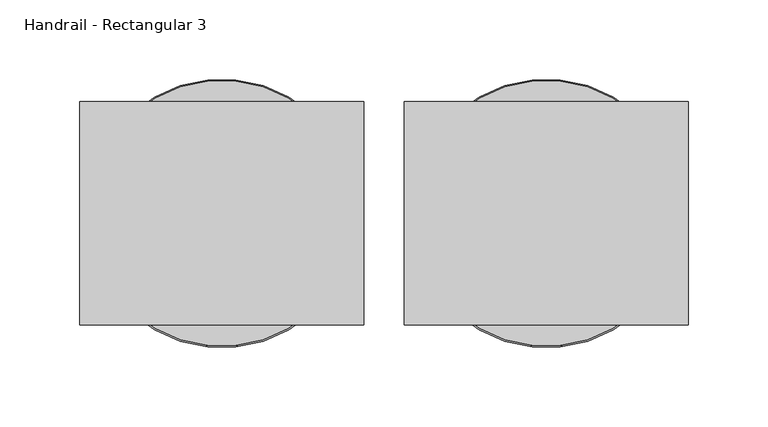
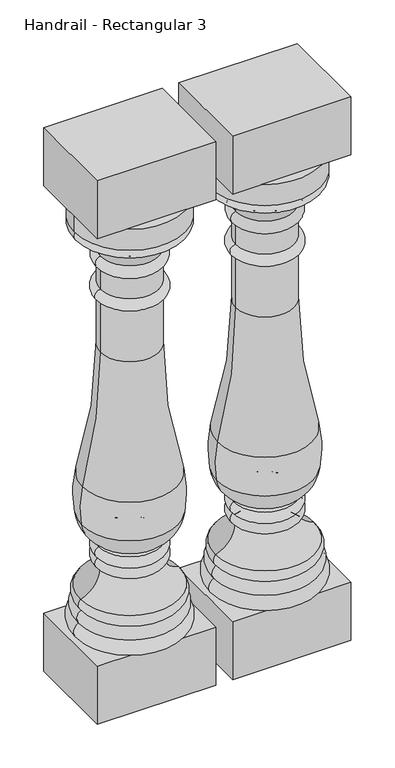
"""IFC4 building model written with IfcOpenShell, lengths in millimetres: railing geometry, Handrail - Rectangular 3."""

from ifc_helpers import new_model, si_unit, point, frame, origin, place, context, project, spatial, polyline, circle_curve, ellipse_curve, trimmed, outline, extrude, source, transform, mapped, element, save
from ifc_brep_helpers import plane_surface, cylinder_surface, revolved_surface, advanced_brep


def handrail_rectangular_3_6060ea51(model_context):
    return source(origin(), model_context, "Body", "SolidModel", [
        advanced_brep(
        [(11610.7084395, -1665.6164768, 849.3125), (11777.3959395, -1665.6164768, 849.3125), (11777.3959395, -1665.6164768, 882.65), (11610.7084395, -1665.6164768, 882.65), (11613.8834395, -1665.6164768, 849.3125), (11774.2209395, -1665.6164768, 849.3125), (11613.8834395, -1665.6164768, 835.025), (11774.2209395, -1665.6164768, 835.025), (11650.3959395, -1665.6164768, 796.925), (11737.7084395, -1665.6164768, 796.925), (11650.3959395, -1665.6164768, 777.875), (11737.7084395, -1665.6164768, 777.875), (11650.3959395, -1665.6164768, 744.5375), (11737.7084395, -1665.6164768, 744.5375), (11650.3959395, -1665.6164768, 727.075), (11737.7084395, -1665.6164768, 727.075), (11650.3959395, -1665.6164768, 644.525), (11737.7084395, -1665.6164768, 644.525), (11623.2074221, -1665.6164768, 440.2065586), (11764.896957, -1665.6164768, 440.2065586), (11622.0170661, -1665.6164768, 379.6643134), (11766.087313, -1665.6164768, 379.6643134), (11649.2281246, -1665.6164768, 340.8286685), (11738.8762545, -1665.6164768, 340.8286685), (11647.5028429, -1665.6164768, 336.3463085), (11740.6015362, -1665.6164768, 336.3463085), (11646.4271895, -1665.6164768, 319.0875), (11741.6771895, -1665.6164768, 319.0875), (11649.6021895, -1665.6164768, 301.625), (11738.5021895, -1665.6164768, 301.625), (11620.2334395, -1665.6164768, 261.9375), (11767.8709395, -1665.6164768, 261.9375), (11621.0271895, -1665.6164768, 244.475), (11767.0771895, -1665.6164768, 244.475), (11617.0584395, -1665.6164768, 225.425), (11771.0459395, -1665.6164768, 225.425), (11613.8834395, -1665.6164768, 203.2), (11774.2209395, -1665.6164768, 203.2), (11694.0521895, -1665.6164768, 203.2), (11694.0521895, -1665.6164768, 882.65)],
        [
            (0, 1, circle_curve(frame((11694.0521895, -1665.6164768, 849.3125), z_axis=(0.0, 0.0, 1.0), x_axis=(1.0, 0.0, 0.0)), 83.34375)),
            (1, 2),
            (2, 3, circle_curve(frame((11694.0521895, -1665.6164768, 882.65), z_axis=(0.0, 0.0, -1.0), x_axis=(1.0, 0.0, 0.0)), 83.34375)),
            (3, 0),
            (1, 0, circle_curve(frame((11694.0521895, -1665.6164768, 849.3125), z_axis=(0.0, 0.0, 1.0), x_axis=(1.0, 0.0, 0.0)), 83.34375)),
            (3, 2, circle_curve(frame((11694.0521895, -1665.6164768, 882.65), z_axis=(0.0, 0.0, -1.0), x_axis=(1.0, 0.0, 0.0)), 83.34375)),
            (4, 5, circle_curve(frame((11694.0521895, -1665.6164768, 849.3125), z_axis=(0.0, 0.0, 1.0), x_axis=(1.0, 0.0, 0.0)), 80.16875)),
            (5, 1),
            (0, 4),
            (5, 4, circle_curve(frame((11694.0521895, -1665.6164768, 849.3125), z_axis=(0.0, 0.0, 1.0), x_axis=(1.0, 0.0, 0.0)), 80.16875)),
            (6, 7, circle_curve(frame((11694.0521895, -1665.6164768, 835.025), z_axis=(0.0, 0.0, 1.0), x_axis=(1.0, 0.0, 0.0)), 80.16875)),
            (7, 5, circle_curve(frame((11767.7717208, -1665.6164768, 842.16875), z_axis=(0.0, -1.0, 0.0), x_axis=(1.0, 0.0, 0.0)), 9.6242187)),
            (4, 6, circle_curve(frame((11620.3326583, -1665.6164768, 842.16875), z_axis=(0.0, -1.0, 0.0), x_axis=(-1.0, 0.0, 0.0)), 9.6242187)),
            (7, 6, circle_curve(frame((11694.0521895, -1665.6164768, 835.025), z_axis=(0.0, 0.0, 1.0), x_axis=(1.0, 0.0, 0.0)), 80.16875)),
            (8, 9, circle_curve(frame((11694.0521895, -1665.6164768, 796.925), z_axis=(0.0, 0.0, 1.0), x_axis=(1.0, 0.0, 0.0)), 43.65625)),
            (9, 7, circle_curve(frame((11793.125244, -1665.6164768, 780.362802), z_axis=(0.0, 1.0, 0.0), x_axis=(1.0, 0.0, 0.0)), 57.8388159)),
            (6, 8, circle_curve(frame((11594.9791351, -1665.6164768, 780.362802), z_axis=(0.0, 1.0, 0.0), x_axis=(-1.0, 0.0, 0.0)), 57.8388159)),
            (9, 8, circle_curve(frame((11694.0521895, -1665.6164768, 796.925), z_axis=(0.0, 0.0, 1.0), x_axis=(1.0, 0.0, 0.0)), 43.65625)),
            (10, 11, circle_curve(frame((11694.0521895, -1665.6164768, 777.875), z_axis=(0.0, 0.0, 1.0), x_axis=(1.0, 0.0, 0.0)), 43.65625)),
            (11, 9, circle_curve(frame((11735.9621895, -1665.6164768, 787.4), z_axis=(0.0, -1.0, 0.0), x_axis=(1.0, 0.0, 0.0)), 9.68375)),
            (8, 10, circle_curve(frame((11652.1421895, -1665.6164768, 787.4), z_axis=(0.0, -1.0, 0.0), x_axis=(-1.0, 0.0, 0.0)), 9.68375)),
            (11, 10, circle_curve(frame((11694.0521895, -1665.6164768, 777.875), z_axis=(0.0, 0.0, 1.0), x_axis=(1.0, 0.0, 0.0)), 43.65625)),
            (12, 13, circle_curve(frame((11694.0521895, -1665.6164768, 744.5375), z_axis=(0.0, 0.0, 1.0), x_axis=(1.0, 0.0, 0.0)), 43.65625)),
            (13, 11),
            (10, 12),
            (13, 12, circle_curve(frame((11694.0521895, -1665.6164768, 744.5375), z_axis=(0.0, 0.0, 1.0), x_axis=(1.0, 0.0, 0.0)), 43.65625)),
            (14, 15, circle_curve(frame((11694.0521895, -1665.6164768, 727.075), z_axis=(0.0, 0.0, 1.0), x_axis=(1.0, 0.0, 0.0)), 43.65625)),
            (15, 13, circle_curve(frame((11737.7084395, -1665.6164768, 735.80625), z_axis=(0.0, -1.0, 0.0), x_axis=(1.0, 0.0, 0.0)), 8.73125)),
            (12, 14, circle_curve(frame((11650.3959395, -1665.6164768, 735.80625), z_axis=(0.0, -1.0, 0.0), x_axis=(-1.0, 0.0, 0.0)), 8.73125)),
            (15, 14, circle_curve(frame((11694.0521895, -1665.6164768, 727.075), z_axis=(0.0, 0.0, 1.0), x_axis=(1.0, 0.0, 0.0)), 43.65625)),
            (16, 17, circle_curve(frame((11694.0521895, -1665.6164768, 644.525), z_axis=(0.0, 0.0, 1.0), x_axis=(1.0, 0.0, 0.0)), 43.65625)),
            (17, 15),
            (14, 16),
            (17, 16, circle_curve(frame((11694.0521895, -1665.6164768, 644.525), z_axis=(0.0, 0.0, 1.0), x_axis=(1.0, 0.0, 0.0)), 43.65625)),
            (18, 19, circle_curve(frame((11694.0521895, -1665.6164768, 440.2065586), z_axis=(0.0, 0.0, 1.0), x_axis=(1.0, 0.0, 0.0)), 70.8447675)),
            (19, 17, circle_curve(frame((12472.4851891, -1665.6164768, 638.333048), z_axis=(0.0, 1.0, 0.0), x_axis=(1.0, 0.0, 0.0)), 734.8028389)),
            (16, 18, circle_curve(frame((10915.61919, -1665.6164768, 638.333048), z_axis=(0.0, 1.0, 0.0), x_axis=(-1.0, 0.0, 0.0)), 734.8028389)),
            (19, 18, circle_curve(frame((11694.0521895, -1665.6164768, 440.2065586), z_axis=(0.0, 0.0, 1.0), x_axis=(1.0, 0.0, 0.0)), 70.8447675)),
            (20, 21, circle_curve(frame((11694.0521895, -1665.6164768, 379.6643134), z_axis=(0.0, 0.0, 1.0), x_axis=(1.0, 0.0, 0.0)), 72.0351235)),
            (21, 19, circle_curve(frame((11606.9983349, -1665.6164768, 406.819198), z_axis=(0.0, -1.0, 0.0), x_axis=(1.0, 0.0, 0.0)), 161.3898718)),
            (18, 20, circle_curve(frame((11781.1060442, -1665.6164768, 406.819198), z_axis=(0.0, -1.0, 0.0), x_axis=(-1.0, 0.0, 0.0)), 161.3898718)),
            (21, 20, circle_curve(frame((11694.0521895, -1665.6164768, 379.6643134), z_axis=(0.0, 0.0, 1.0), x_axis=(1.0, 0.0, 0.0)), 72.0351235)),
            (22, 23, circle_curve(frame((11694.0521895, -1665.6164768, 340.8286685), z_axis=(0.0, 0.0, 1.0), x_axis=(1.0, 0.0, 0.0)), 44.8240649)),
            (23, 21, circle_curve(frame((11716.3572912, -1665.6164768, 385.5579203), z_axis=(0.0, -1.0, 0.0), x_axis=(1.0, 0.0, 0.0)), 50.0780358)),
            (20, 22, circle_curve(frame((11671.7470879, -1665.6164768, 385.5579203), z_axis=(0.0, -1.0, 0.0), x_axis=(-1.0, 0.0, 0.0)), 50.0780358)),
            (23, 22, circle_curve(frame((11694.0521895, -1665.6164768, 340.8286685), z_axis=(0.0, 0.0, 1.0), x_axis=(1.0, 0.0, 0.0)), 44.8240649)),
            (24, 25, circle_curve(frame((11694.0521895, -1665.6164768, 336.3463085), z_axis=(0.0, 0.0, 1.0), x_axis=(1.0, 0.0, 0.0)), 46.5493467)),
            (25, 23, circle_curve(frame((11741.6771895, -1665.6164768, 339.3335472), z_axis=(0.0, 1.0, 0.0), x_axis=(1.0, 0.0, 0.0)), 3.175)),
            (22, 24, circle_curve(frame((11646.4271895, -1665.6164768, 339.3335472), z_axis=(0.0, 1.0, 0.0), x_axis=(-1.0, 0.0, 0.0)), 3.175)),
            (25, 24, circle_curve(frame((11694.0521895, -1665.6164768, 336.3463085), z_axis=(0.0, 0.0, 1.0), x_axis=(1.0, 0.0, 0.0)), 46.5493467)),
            (26, 27, circle_curve(frame((11694.0521895, -1665.6164768, 319.0875), z_axis=(0.0, 0.0, 1.0), x_axis=(1.0, 0.0, 0.0)), 47.625)),
            (27, 25, circle_curve(frame((11736.6008248, -1665.6164768, 327.4340404), z_axis=(0.0, -1.0, 0.0), x_axis=(1.0, 0.0, 0.0)), 9.7690437)),
            (24, 26, circle_curve(frame((11651.5035543, -1665.6164768, 327.4340404), z_axis=(0.0, -1.0, 0.0), x_axis=(-1.0, 0.0, 0.0)), 9.7690437)),
            (27, 26, circle_curve(frame((11694.0521895, -1665.6164768, 319.0875), z_axis=(0.0, 0.0, 1.0), x_axis=(1.0, 0.0, 0.0)), 47.625)),
            (28, 29, circle_curve(frame((11694.0521895, -1665.6164768, 301.625), z_axis=(0.0, 0.0, 1.0), x_axis=(1.0, 0.0, 0.0)), 44.45)),
            (29, 27, circle_curve(frame((11737.0635177, -1665.6164768, 310.9064631), z_axis=(0.0, -1.0, 0.0), x_axis=(1.0, 0.0, 0.0)), 9.3923018)),
            (26, 28, circle_curve(frame((11651.0408614, -1665.6164768, 310.9064631), z_axis=(0.0, -1.0, 0.0), x_axis=(-1.0, 0.0, 0.0)), 9.3923018)),
            (29, 28, circle_curve(frame((11694.0521895, -1665.6164768, 301.625), z_axis=(0.0, 0.0, 1.0), x_axis=(1.0, 0.0, 0.0)), 44.45)),
            (30, 31, circle_curve(frame((11694.0521895, -1665.6164768, 261.9375), z_axis=(0.0, 0.0, 1.0), x_axis=(1.0, 0.0, 0.0)), 73.81875)),
            (31, 29, circle_curve(frame((11780.0024429, -1665.6164768, 301.625), z_axis=(0.0, 1.0, 0.0), x_axis=(1.0, 0.0, 0.0)), 41.5002534)),
            (28, 30, circle_curve(frame((11608.1019362, -1665.6164768, 301.625), z_axis=(0.0, 1.0, 0.0), x_axis=(-1.0, 0.0, 0.0)), 41.5002534)),
            (31, 30, circle_curve(frame((11694.0521895, -1665.6164768, 261.9375), z_axis=(0.0, 0.0, 1.0), x_axis=(1.0, 0.0, 0.0)), 73.81875)),
            (32, 33, circle_curve(frame((11694.0521895, -1665.6164768, 244.475), z_axis=(0.0, 0.0, 1.0), x_axis=(1.0, 0.0, 0.0)), 73.025)),
            (33, 31, circle_curve(frame((11758.5664257, -1665.6164768, 253.6111427), z_axis=(0.0, -1.0, 0.0), x_axis=(1.0, 0.0, 0.0)), 12.4860804)),
            (30, 32, circle_curve(frame((11629.5379534, -1665.6164768, 253.6111427), z_axis=(0.0, -1.0, 0.0), x_axis=(-1.0, 0.0, 0.0)), 12.4860804)),
            (33, 32, circle_curve(frame((11694.0521895, -1665.6164768, 244.475), z_axis=(0.0, 0.0, 1.0), x_axis=(1.0, 0.0, 0.0)), 73.025)),
            (34, 35, circle_curve(frame((11694.0521895, -1665.6164768, 225.425), z_axis=(0.0, 0.0, 1.0), x_axis=(1.0, 0.0, 0.0)), 76.99375)),
            (35, 33, circle_curve(frame((11760.4024736, -1665.6164768, 233.1460227), z_axis=(0.0, -1.0, 0.0), x_axis=(1.0, 0.0, 0.0)), 13.1490516)),
            (32, 34, circle_curve(frame((11627.7019054, -1665.6164768, 233.1460227), z_axis=(0.0, -1.0, 0.0), x_axis=(-1.0, 0.0, 0.0)), 13.1490516)),
            (35, 34, circle_curve(frame((11694.0521895, -1665.6164768, 225.425), z_axis=(0.0, 0.0, 1.0), x_axis=(1.0, 0.0, 0.0)), 76.99375)),
            (36, 37, circle_curve(frame((11694.0521895, -1665.6164768, 203.2), z_axis=(0.0, 0.0, 1.0), x_axis=(1.0, 0.0, 0.0)), 80.16875)),
            (37, 35, circle_curve(frame((11764.0722788, -1665.6164768, 213.089477), z_axis=(0.0, -1.0, 0.0), x_axis=(1.0, 0.0, 0.0)), 14.1702883)),
            (34, 36, circle_curve(frame((11624.0321003, -1665.6164768, 213.089477), z_axis=(0.0, -1.0, 0.0), x_axis=(-1.0, 0.0, 0.0)), 14.1702883)),
            (37, 36, circle_curve(frame((11694.0521895, -1665.6164768, 203.2), z_axis=(0.0, 0.0, 1.0), x_axis=(1.0, 0.0, 0.0)), 80.16875)),
            (38, 37),
            (36, 38),
            (2, 39),
            (39, 3),
        ],
        [
            cylinder_surface(frame((11694.0521895, -1665.6164768, 831.85), z_axis=(0.0, 0.0, -1.0), x_axis=(1.0, 0.0, 0.0)), 83.34375),
            plane_surface(frame((11694.0521895, -1665.6164768, 849.3125), z_axis=(0.0, 0.0, -1.0), x_axis=(1.0, 0.0, 0.0))),
            revolved_surface(trimmed(ellipse_curve(frame((11767.7717208, -1665.6164768, 842.16875), z_axis=(0.0, 1.0, 0.0), x_axis=(1.0, 0.0, 0.0)), 9.6242187, 9.6242187), [point((11774.2209395, -1665.6164768, 849.3125))], [point((11774.2209395, -1665.6164768, 835.025))], True, "CARTESIAN"), (11694.0521895, -1665.6164768, 831.85), (0.0, 0.0, -1.0)),
            revolved_surface(trimmed(ellipse_curve(frame((11793.125244, -1665.6164768, 780.362802), z_axis=(0.0, -1.0, 0.0), x_axis=(1.0, 0.0, 0.0)), 57.8388159, 57.8388159), [point((11774.2209395, -1665.6164768, 835.025))], [point((11737.7084395, -1665.6164768, 796.925))], True, "CARTESIAN"), (11694.0521895, -1665.6164768, 831.85), (0.0, 0.0, -1.0)),
            revolved_surface(trimmed(ellipse_curve(frame((11735.9621895, -1665.6164768, 787.4), z_axis=(0.0, 1.0, 0.0), x_axis=(1.0, 0.0, 0.0)), 9.68375, 9.68375), [point((11737.7084395, -1665.6164768, 796.925))], [point((11737.7084395, -1665.6164768, 777.875))], True, "CARTESIAN"), (11694.0521895, -1665.6164768, 831.85), (0.0, 0.0, -1.0)),
            cylinder_surface(frame((11694.0521895, -1665.6164768, 831.85), z_axis=(0.0, 0.0, -1.0), x_axis=(1.0, 0.0, 0.0)), 43.65625),
            revolved_surface(trimmed(ellipse_curve(frame((11737.7084395, -1665.6164768, 735.80625), z_axis=(0.0, 1.0, 0.0), x_axis=(1.0, 0.0, 0.0)), 8.73125, 8.73125), [point((11737.7084395, -1665.6164768, 744.5375))], [point((11737.7084395, -1665.6164768, 727.075))], True, "CARTESIAN"), (11694.0521895, -1665.6164768, 831.85), (0.0, 0.0, -1.0)),
            revolved_surface(trimmed(ellipse_curve(frame((12472.4851891, -1665.6164768, 638.333048), z_axis=(0.0, -1.0, 0.0), x_axis=(1.0, 0.0, 0.0)), 734.8028389, 734.8028389), [point((11737.7084395, -1665.6164768, 644.525))], [point((11764.896957, -1665.6164768, 440.2065586))], True, "CARTESIAN"), (11694.0521895, -1665.6164768, 831.85), (0.0, 0.0, -1.0)),
            revolved_surface(trimmed(ellipse_curve(frame((11606.9983349, -1665.6164768, 406.819198), z_axis=(0.0, 1.0, 0.0), x_axis=(1.0, 0.0, 0.0)), 161.3898718, 161.3898718), [point((11764.896957, -1665.6164768, 440.2065586))], [point((11766.087313, -1665.6164768, 379.6643134))], True, "CARTESIAN"), (11694.0521895, -1665.6164768, 831.85), (0.0, 0.0, -1.0)),
            revolved_surface(trimmed(ellipse_curve(frame((11716.3572912, -1665.6164768, 385.5579203), z_axis=(0.0, 1.0, 0.0), x_axis=(1.0, 0.0, 0.0)), 50.0780358, 50.0780358), [point((11766.087313, -1665.6164768, 379.6643134))], [point((11738.8762545, -1665.6164768, 340.8286685))], True, "CARTESIAN"), (11694.0521895, -1665.6164768, 831.85), (0.0, 0.0, -1.0)),
            revolved_surface(trimmed(ellipse_curve(frame((11741.6771895, -1665.6164768, 339.3335472), z_axis=(0.0, -1.0, 0.0), x_axis=(1.0, 0.0, 0.0)), 3.175, 3.175), [point((11738.8762545, -1665.6164768, 340.8286685))], [point((11740.6015362, -1665.6164768, 336.3463085))], True, "CARTESIAN"), (11694.0521895, -1665.6164768, 831.85), (0.0, 0.0, -1.0)),
            revolved_surface(trimmed(ellipse_curve(frame((11736.6008248, -1665.6164768, 327.4340404), z_axis=(0.0, 1.0, 0.0), x_axis=(1.0, 0.0, 0.0)), 9.7690437, 9.7690437), [point((11740.6015362, -1665.6164768, 336.3463085))], [point((11741.6771895, -1665.6164768, 319.0875))], True, "CARTESIAN"), (11694.0521895, -1665.6164768, 831.85), (0.0, 0.0, -1.0)),
            revolved_surface(trimmed(ellipse_curve(frame((11737.0635177, -1665.6164768, 310.9064631), z_axis=(0.0, 1.0, 0.0), x_axis=(1.0, 0.0, 0.0)), 9.3923018, 9.3923018), [point((11741.6771895, -1665.6164768, 319.0875))], [point((11738.5021895, -1665.6164768, 301.625))], True, "CARTESIAN"), (11694.0521895, -1665.6164768, 831.85), (0.0, 0.0, -1.0)),
            revolved_surface(trimmed(ellipse_curve(frame((11780.0024429, -1665.6164768, 301.625), z_axis=(0.0, -1.0, 0.0), x_axis=(1.0, 0.0, 0.0)), 41.5002534, 41.5002534), [point((11738.5021895, -1665.6164768, 301.625))], [point((11767.8709395, -1665.6164768, 261.9375))], True, "CARTESIAN"), (11694.0521895, -1665.6164768, 831.85), (0.0, 0.0, -1.0)),
            revolved_surface(trimmed(ellipse_curve(frame((11758.5664257, -1665.6164768, 253.6111427), z_axis=(0.0, 1.0, 0.0), x_axis=(1.0, 0.0, 0.0)), 12.4860804, 12.4860804), [point((11767.8709395, -1665.6164768, 261.9375))], [point((11767.0771895, -1665.6164768, 244.475))], True, "CARTESIAN"), (11694.0521895, -1665.6164768, 831.85), (0.0, 0.0, -1.0)),
            revolved_surface(trimmed(ellipse_curve(frame((11760.4024736, -1665.6164768, 233.1460227), z_axis=(0.0, 1.0, 0.0), x_axis=(1.0, 0.0, 0.0)), 13.1490516, 13.1490516), [point((11767.0771895, -1665.6164768, 244.475))], [point((11771.0459395, -1665.6164768, 225.425))], True, "CARTESIAN"), (11694.0521895, -1665.6164768, 831.85), (0.0, 0.0, -1.0)),
            revolved_surface(trimmed(ellipse_curve(frame((11764.0722788, -1665.6164768, 213.089477), z_axis=(0.0, 1.0, 0.0), x_axis=(1.0, 0.0, 0.0)), 14.1702883, 14.1702883), [point((11771.0459395, -1665.6164768, 225.425))], [point((11774.2209395, -1665.6164768, 203.2))], True, "CARTESIAN"), (11694.0521895, -1665.6164768, 831.85), (0.0, 0.0, -1.0)),
            plane_surface(frame((11694.0521895, -1665.6164768, 203.2), z_axis=(0.0, 0.0, -1.0), x_axis=(1.0, 0.0, 0.0))),
            plane_surface(frame((11694.0521895, -1665.6164768, 882.65), z_axis=(0.0, 0.0, 1.0), x_axis=(1.0, 0.0, 0.0))),
        ],
        [
            (0, [[1, 2, 3, 4]]),
            (0, [[5, -4, 6, -2]]),
            (1, [[7, 8, -1, 9]]),
            (1, [[10, -9, -5, -8]]),
            (2, [[11, 12, -7, 13]]),
            (2, [[14, -13, -10, -12]]),
            (3, [[15, 16, -11, 17]]),
            (3, [[18, -17, -14, -16]]),
            (4, [[19, 20, -15, 21]]),
            (4, [[22, -21, -18, -20]]),
            (5, [[23, 24, -19, 25]]),
            (5, [[26, -25, -22, -24]]),
            (6, [[27, 28, -23, 29]]),
            (6, [[30, -29, -26, -28]]),
            (5, [[31, 32, -27, 33]]),
            (5, [[34, -33, -30, -32]]),
            (7, [[35, 36, -31, 37]]),
            (7, [[38, -37, -34, -36]]),
            (8, [[39, 40, -35, 41]]),
            (8, [[42, -41, -38, -40]]),
            (9, [[43, 44, -39, 45]]),
            (9, [[46, -45, -42, -44]]),
            (10, [[47, 48, -43, 49]]),
            (10, [[50, -49, -46, -48]]),
            (11, [[51, 52, -47, 53]]),
            (11, [[54, -53, -50, -52]]),
            (12, [[55, 56, -51, 57]]),
            (12, [[58, -57, -54, -56]]),
            (13, [[59, 60, -55, 61]]),
            (13, [[62, -61, -58, -60]]),
            (14, [[63, 64, -59, 65]]),
            (14, [[66, -65, -62, -64]]),
            (15, [[67, 68, -63, 69]]),
            (15, [[70, -69, -66, -68]]),
            (16, [[71, 72, -67, 73]]),
            (16, [[74, -73, -70, -72]]),
            (17, [[75, -71, 76]]),
            (17, [[-76, -74, -75]]),
            (18, [[-3, 77, 78]]),
            (18, [[-6, -78, -77]]),
        ],
    ),
        extrude(outline(polyline([(11605.1521895, -1735.4664768), (11605.1521895, -1595.7664768), (11782.9521895, -1595.7664768), (11782.9521895, -1735.4664768), (11605.1521895, -1735.4664768)])), frame((0.0, 0.0, 111.125), z_axis=(0.0, 0.0, 1.0), x_axis=(1.0, 0.0, 0.0)), (0.0, 0.0, 1.0), 92.075),
        extrude(outline(polyline([(11605.1521895, -1595.7664768), (11782.9521895, -1595.7664768), (11782.9521895, -1735.4664768), (11605.1521895, -1735.4664768), (11605.1521895, -1595.7664768)])), frame((0.0, 0.0, 882.65), z_axis=(0.0, 0.0, 1.0), x_axis=(1.0, 0.0, 0.0)), (0.0, 0.0, 1.0), 92.075),
        advanced_brep(
        [(11407.5084395, -1665.6164768, 849.3125), (11574.1959395, -1665.6164768, 849.3125), (11574.1959395, -1665.6164768, 882.65), (11407.5084395, -1665.6164768, 882.65), (11410.6834395, -1665.6164768, 849.3125), (11571.0209395, -1665.6164768, 849.3125), (11410.6834395, -1665.6164768, 835.025), (11571.0209395, -1665.6164768, 835.025), (11447.1959395, -1665.6164768, 796.925), (11534.5084395, -1665.6164768, 796.925), (11447.1959395, -1665.6164768, 777.875), (11534.5084395, -1665.6164768, 777.875), (11447.1959395, -1665.6164768, 744.5375), (11534.5084395, -1665.6164768, 744.5375), (11447.1959395, -1665.6164768, 727.075), (11534.5084395, -1665.6164768, 727.075), (11447.1959395, -1665.6164768, 644.525), (11534.5084395, -1665.6164768, 644.525), (11420.0074221, -1665.6164768, 440.2065586), (11561.696957, -1665.6164768, 440.2065586), (11418.8170661, -1665.6164768, 379.6643134), (11562.887313, -1665.6164768, 379.6643134), (11446.0281246, -1665.6164768, 340.8286685), (11535.6762545, -1665.6164768, 340.8286685), (11444.3028429, -1665.6164768, 336.3463085), (11537.4015362, -1665.6164768, 336.3463085), (11443.2271895, -1665.6164768, 319.0875), (11538.4771895, -1665.6164768, 319.0875), (11446.4021895, -1665.6164768, 301.625), (11535.3021895, -1665.6164768, 301.625), (11417.0334395, -1665.6164768, 261.9375), (11564.6709395, -1665.6164768, 261.9375), (11417.8271895, -1665.6164768, 244.475), (11563.8771895, -1665.6164768, 244.475), (11413.8584395, -1665.6164768, 225.425), (11567.8459395, -1665.6164768, 225.425), (11410.6834395, -1665.6164768, 203.2), (11571.0209395, -1665.6164768, 203.2), (11490.8521895, -1665.6164768, 203.2), (11490.8521895, -1665.6164768, 882.65)],
        [
            (0, 1, circle_curve(frame((11490.8521895, -1665.6164768, 849.3125), z_axis=(0.0, 0.0, 1.0), x_axis=(1.0, 0.0, 0.0)), 83.34375)),
            (1, 2),
            (2, 3, circle_curve(frame((11490.8521895, -1665.6164768, 882.65), z_axis=(0.0, 0.0, -1.0), x_axis=(1.0, 0.0, 0.0)), 83.34375)),
            (3, 0),
            (1, 0, circle_curve(frame((11490.8521895, -1665.6164768, 849.3125), z_axis=(0.0, 0.0, 1.0), x_axis=(1.0, 0.0, 0.0)), 83.34375)),
            (3, 2, circle_curve(frame((11490.8521895, -1665.6164768, 882.65), z_axis=(0.0, 0.0, -1.0), x_axis=(1.0, 0.0, 0.0)), 83.34375)),
            (4, 5, circle_curve(frame((11490.8521895, -1665.6164768, 849.3125), z_axis=(0.0, 0.0, 1.0), x_axis=(1.0, 0.0, 0.0)), 80.16875)),
            (5, 1),
            (0, 4),
            (5, 4, circle_curve(frame((11490.8521895, -1665.6164768, 849.3125), z_axis=(0.0, 0.0, 1.0), x_axis=(1.0, 0.0, 0.0)), 80.16875)),
            (6, 7, circle_curve(frame((11490.8521895, -1665.6164768, 835.025), z_axis=(0.0, 0.0, 1.0), x_axis=(1.0, 0.0, 0.0)), 80.16875)),
            (7, 5, circle_curve(frame((11564.5717208, -1665.6164768, 842.16875), z_axis=(0.0, -1.0, 0.0), x_axis=(1.0, 0.0, 0.0)), 9.6242187)),
            (4, 6, circle_curve(frame((11417.1326583, -1665.6164768, 842.16875), z_axis=(0.0, -1.0, 0.0), x_axis=(-1.0, 0.0, 0.0)), 9.6242187)),
            (7, 6, circle_curve(frame((11490.8521895, -1665.6164768, 835.025), z_axis=(0.0, 0.0, 1.0), x_axis=(1.0, 0.0, 0.0)), 80.16875)),
            (8, 9, circle_curve(frame((11490.8521895, -1665.6164768, 796.925), z_axis=(0.0, 0.0, 1.0), x_axis=(1.0, 0.0, 0.0)), 43.65625)),
            (9, 7, circle_curve(frame((11589.925244, -1665.6164768, 780.362802), z_axis=(0.0, 1.0, 0.0), x_axis=(1.0, 0.0, 0.0)), 57.8388159)),
            (6, 8, circle_curve(frame((11391.7791351, -1665.6164768, 780.362802), z_axis=(0.0, 1.0, 0.0), x_axis=(-1.0, 0.0, 0.0)), 57.8388159)),
            (9, 8, circle_curve(frame((11490.8521895, -1665.6164768, 796.925), z_axis=(0.0, 0.0, 1.0), x_axis=(1.0, 0.0, 0.0)), 43.65625)),
            (10, 11, circle_curve(frame((11490.8521895, -1665.6164768, 777.875), z_axis=(0.0, 0.0, 1.0), x_axis=(1.0, 0.0, 0.0)), 43.65625)),
            (11, 9, circle_curve(frame((11532.7621895, -1665.6164768, 787.4), z_axis=(0.0, -1.0, 0.0), x_axis=(1.0, 0.0, 0.0)), 9.68375)),
            (8, 10, circle_curve(frame((11448.9421895, -1665.6164768, 787.4), z_axis=(0.0, -1.0, 0.0), x_axis=(-1.0, 0.0, 0.0)), 9.68375)),
            (11, 10, circle_curve(frame((11490.8521895, -1665.6164768, 777.875), z_axis=(0.0, 0.0, 1.0), x_axis=(1.0, 0.0, 0.0)), 43.65625)),
            (12, 13, circle_curve(frame((11490.8521895, -1665.6164768, 744.5375), z_axis=(0.0, 0.0, 1.0), x_axis=(1.0, 0.0, 0.0)), 43.65625)),
            (13, 11),
            (10, 12),
            (13, 12, circle_curve(frame((11490.8521895, -1665.6164768, 744.5375), z_axis=(0.0, 0.0, 1.0), x_axis=(1.0, 0.0, 0.0)), 43.65625)),
            (14, 15, circle_curve(frame((11490.8521895, -1665.6164768, 727.075), z_axis=(0.0, 0.0, 1.0), x_axis=(1.0, 0.0, 0.0)), 43.65625)),
            (15, 13, circle_curve(frame((11534.5084395, -1665.6164768, 735.80625), z_axis=(0.0, -1.0, 0.0), x_axis=(1.0, 0.0, 0.0)), 8.73125)),
            (12, 14, circle_curve(frame((11447.1959395, -1665.6164768, 735.80625), z_axis=(0.0, -1.0, 0.0), x_axis=(-1.0, 0.0, 0.0)), 8.73125)),
            (15, 14, circle_curve(frame((11490.8521895, -1665.6164768, 727.075), z_axis=(0.0, 0.0, 1.0), x_axis=(1.0, 0.0, 0.0)), 43.65625)),
            (16, 17, circle_curve(frame((11490.8521895, -1665.6164768, 644.525), z_axis=(0.0, 0.0, 1.0), x_axis=(1.0, 0.0, 0.0)), 43.65625)),
            (17, 15),
            (14, 16),
            (17, 16, circle_curve(frame((11490.8521895, -1665.6164768, 644.525), z_axis=(0.0, 0.0, 1.0), x_axis=(1.0, 0.0, 0.0)), 43.65625)),
            (18, 19, circle_curve(frame((11490.8521895, -1665.6164768, 440.2065586), z_axis=(0.0, 0.0, 1.0), x_axis=(1.0, 0.0, 0.0)), 70.8447675)),
            (19, 17, circle_curve(frame((12269.2851891, -1665.6164768, 638.333048), z_axis=(0.0, 1.0, 0.0), x_axis=(1.0, 0.0, 0.0)), 734.8028389)),
            (16, 18, circle_curve(frame((10712.41919, -1665.6164768, 638.333048), z_axis=(0.0, 1.0, 0.0), x_axis=(-1.0, 0.0, 0.0)), 734.8028389)),
            (19, 18, circle_curve(frame((11490.8521895, -1665.6164768, 440.2065586), z_axis=(0.0, 0.0, 1.0), x_axis=(1.0, 0.0, 0.0)), 70.8447675)),
            (20, 21, circle_curve(frame((11490.8521895, -1665.6164768, 379.6643134), z_axis=(0.0, 0.0, 1.0), x_axis=(1.0, 0.0, 0.0)), 72.0351235)),
            (21, 19, circle_curve(frame((11403.7983349, -1665.6164768, 406.819198), z_axis=(0.0, -1.0, 0.0), x_axis=(1.0, 0.0, 0.0)), 161.3898718)),
            (18, 20, circle_curve(frame((11577.9060442, -1665.6164768, 406.819198), z_axis=(0.0, -1.0, 0.0), x_axis=(-1.0, 0.0, 0.0)), 161.3898718)),
            (21, 20, circle_curve(frame((11490.8521895, -1665.6164768, 379.6643134), z_axis=(0.0, 0.0, 1.0), x_axis=(1.0, 0.0, 0.0)), 72.0351235)),
            (22, 23, circle_curve(frame((11490.8521895, -1665.6164768, 340.8286685), z_axis=(0.0, 0.0, 1.0), x_axis=(1.0, 0.0, 0.0)), 44.8240649)),
            (23, 21, circle_curve(frame((11513.1572912, -1665.6164768, 385.5579203), z_axis=(0.0, -1.0, 0.0), x_axis=(1.0, 0.0, 0.0)), 50.0780358)),
            (20, 22, circle_curve(frame((11468.5470879, -1665.6164768, 385.5579203), z_axis=(0.0, -1.0, 0.0), x_axis=(-1.0, 0.0, 0.0)), 50.0780358)),
            (23, 22, circle_curve(frame((11490.8521895, -1665.6164768, 340.8286685), z_axis=(0.0, 0.0, 1.0), x_axis=(1.0, 0.0, 0.0)), 44.8240649)),
            (24, 25, circle_curve(frame((11490.8521895, -1665.6164768, 336.3463085), z_axis=(0.0, 0.0, 1.0), x_axis=(1.0, 0.0, 0.0)), 46.5493467)),
            (25, 23, circle_curve(frame((11538.4771895, -1665.6164768, 339.3335472), z_axis=(0.0, 1.0, 0.0), x_axis=(1.0, 0.0, 0.0)), 3.175)),
            (22, 24, circle_curve(frame((11443.2271895, -1665.6164768, 339.3335472), z_axis=(0.0, 1.0, 0.0), x_axis=(-1.0, 0.0, 0.0)), 3.175)),
            (25, 24, circle_curve(frame((11490.8521895, -1665.6164768, 336.3463085), z_axis=(0.0, 0.0, 1.0), x_axis=(1.0, 0.0, 0.0)), 46.5493467)),
            (26, 27, circle_curve(frame((11490.8521895, -1665.6164768, 319.0875), z_axis=(0.0, 0.0, 1.0), x_axis=(1.0, 0.0, 0.0)), 47.625)),
            (27, 25, circle_curve(frame((11533.4008248, -1665.6164768, 327.4340404), z_axis=(0.0, -1.0, 0.0), x_axis=(1.0, 0.0, 0.0)), 9.7690437)),
            (24, 26, circle_curve(frame((11448.3035543, -1665.6164768, 327.4340404), z_axis=(0.0, -1.0, 0.0), x_axis=(-1.0, 0.0, 0.0)), 9.7690437)),
            (27, 26, circle_curve(frame((11490.8521895, -1665.6164768, 319.0875), z_axis=(0.0, 0.0, 1.0), x_axis=(1.0, 0.0, 0.0)), 47.625)),
            (28, 29, circle_curve(frame((11490.8521895, -1665.6164768, 301.625), z_axis=(0.0, 0.0, 1.0), x_axis=(1.0, 0.0, 0.0)), 44.45)),
            (29, 27, circle_curve(frame((11533.8635177, -1665.6164768, 310.9064631), z_axis=(0.0, -1.0, 0.0), x_axis=(1.0, 0.0, 0.0)), 9.3923018)),
            (26, 28, circle_curve(frame((11447.8408614, -1665.6164768, 310.9064631), z_axis=(0.0, -1.0, 0.0), x_axis=(-1.0, 0.0, 0.0)), 9.3923018)),
            (29, 28, circle_curve(frame((11490.8521895, -1665.6164768, 301.625), z_axis=(0.0, 0.0, 1.0), x_axis=(1.0, 0.0, 0.0)), 44.45)),
            (30, 31, circle_curve(frame((11490.8521895, -1665.6164768, 261.9375), z_axis=(0.0, 0.0, 1.0), x_axis=(1.0, 0.0, 0.0)), 73.81875)),
            (31, 29, circle_curve(frame((11576.8024429, -1665.6164768, 301.625), z_axis=(0.0, 1.0, 0.0), x_axis=(1.0, 0.0, 0.0)), 41.5002534)),
            (28, 30, circle_curve(frame((11404.9019362, -1665.6164768, 301.625), z_axis=(0.0, 1.0, 0.0), x_axis=(-1.0, 0.0, 0.0)), 41.5002534)),
            (31, 30, circle_curve(frame((11490.8521895, -1665.6164768, 261.9375), z_axis=(0.0, 0.0, 1.0), x_axis=(1.0, 0.0, 0.0)), 73.81875)),
            (32, 33, circle_curve(frame((11490.8521895, -1665.6164768, 244.475), z_axis=(0.0, 0.0, 1.0), x_axis=(1.0, 0.0, 0.0)), 73.025)),
            (33, 31, circle_curve(frame((11555.3664257, -1665.6164768, 253.6111427), z_axis=(0.0, -1.0, 0.0), x_axis=(1.0, 0.0, 0.0)), 12.4860804)),
            (30, 32, circle_curve(frame((11426.3379534, -1665.6164768, 253.6111427), z_axis=(0.0, -1.0, 0.0), x_axis=(-1.0, 0.0, 0.0)), 12.4860804)),
            (33, 32, circle_curve(frame((11490.8521895, -1665.6164768, 244.475), z_axis=(0.0, 0.0, 1.0), x_axis=(1.0, 0.0, 0.0)), 73.025)),
            (34, 35, circle_curve(frame((11490.8521895, -1665.6164768, 225.425), z_axis=(0.0, 0.0, 1.0), x_axis=(1.0, 0.0, 0.0)), 76.99375)),
            (35, 33, circle_curve(frame((11557.2024736, -1665.6164768, 233.1460227), z_axis=(0.0, -1.0, 0.0), x_axis=(1.0, 0.0, 0.0)), 13.1490516)),
            (32, 34, circle_curve(frame((11424.5019054, -1665.6164768, 233.1460227), z_axis=(0.0, -1.0, 0.0), x_axis=(-1.0, 0.0, 0.0)), 13.1490516)),
            (35, 34, circle_curve(frame((11490.8521895, -1665.6164768, 225.425), z_axis=(0.0, 0.0, 1.0), x_axis=(1.0, 0.0, 0.0)), 76.99375)),
            (36, 37, circle_curve(frame((11490.8521895, -1665.6164768, 203.2), z_axis=(0.0, 0.0, 1.0), x_axis=(1.0, 0.0, 0.0)), 80.16875)),
            (37, 35, circle_curve(frame((11560.8722788, -1665.6164768, 213.089477), z_axis=(0.0, -1.0, 0.0), x_axis=(1.0, 0.0, 0.0)), 14.1702883)),
            (34, 36, circle_curve(frame((11420.8321003, -1665.6164768, 213.089477), z_axis=(0.0, -1.0, 0.0), x_axis=(-1.0, 0.0, 0.0)), 14.1702883)),
            (37, 36, circle_curve(frame((11490.8521895, -1665.6164768, 203.2), z_axis=(0.0, 0.0, 1.0), x_axis=(1.0, 0.0, 0.0)), 80.16875)),
            (38, 37),
            (36, 38),
            (2, 39),
            (39, 3),
        ],
        [
            cylinder_surface(frame((11490.8521895, -1665.6164768, 831.85), z_axis=(0.0, 0.0, -1.0), x_axis=(1.0, 0.0, 0.0)), 83.34375),
            plane_surface(frame((11490.8521895, -1665.6164768, 849.3125), z_axis=(0.0, 0.0, -1.0), x_axis=(1.0, 0.0, 0.0))),
            revolved_surface(trimmed(ellipse_curve(frame((11564.5717208, -1665.6164768, 842.16875), z_axis=(0.0, 1.0, 0.0), x_axis=(1.0, 0.0, 0.0)), 9.6242187, 9.6242187), [point((11571.0209395, -1665.6164768, 849.3125))], [point((11571.0209395, -1665.6164768, 835.025))], True, "CARTESIAN"), (11490.8521895, -1665.6164768, 831.85), (0.0, 0.0, -1.0)),
            revolved_surface(trimmed(ellipse_curve(frame((11589.925244, -1665.6164768, 780.362802), z_axis=(0.0, -1.0, 0.0), x_axis=(1.0, 0.0, 0.0)), 57.8388159, 57.8388159), [point((11571.0209395, -1665.6164768, 835.025))], [point((11534.5084395, -1665.6164768, 796.925))], True, "CARTESIAN"), (11490.8521895, -1665.6164768, 831.85), (0.0, 0.0, -1.0)),
            revolved_surface(trimmed(ellipse_curve(frame((11532.7621895, -1665.6164768, 787.4), z_axis=(0.0, 1.0, 0.0), x_axis=(1.0, 0.0, 0.0)), 9.68375, 9.68375), [point((11534.5084395, -1665.6164768, 796.925))], [point((11534.5084395, -1665.6164768, 777.875))], True, "CARTESIAN"), (11490.8521895, -1665.6164768, 831.85), (0.0, 0.0, -1.0)),
            cylinder_surface(frame((11490.8521895, -1665.6164768, 831.85), z_axis=(0.0, 0.0, -1.0), x_axis=(1.0, 0.0, 0.0)), 43.65625),
            revolved_surface(trimmed(ellipse_curve(frame((11534.5084395, -1665.6164768, 735.80625), z_axis=(0.0, 1.0, 0.0), x_axis=(1.0, 0.0, 0.0)), 8.73125, 8.73125), [point((11534.5084395, -1665.6164768, 744.5375))], [point((11534.5084395, -1665.6164768, 727.075))], True, "CARTESIAN"), (11490.8521895, -1665.6164768, 831.85), (0.0, 0.0, -1.0)),
            revolved_surface(trimmed(ellipse_curve(frame((12269.2851891, -1665.6164768, 638.333048), z_axis=(0.0, -1.0, 0.0), x_axis=(1.0, 0.0, 0.0)), 734.8028389, 734.8028389), [point((11534.5084395, -1665.6164768, 644.525))], [point((11561.696957, -1665.6164768, 440.2065586))], True, "CARTESIAN"), (11490.8521895, -1665.6164768, 831.85), (0.0, 0.0, -1.0)),
            revolved_surface(trimmed(ellipse_curve(frame((11403.7983349, -1665.6164768, 406.819198), z_axis=(0.0, 1.0, 0.0), x_axis=(1.0, 0.0, 0.0)), 161.3898718, 161.3898718), [point((11561.696957, -1665.6164768, 440.2065586))], [point((11562.887313, -1665.6164768, 379.6643134))], True, "CARTESIAN"), (11490.8521895, -1665.6164768, 831.85), (0.0, 0.0, -1.0)),
            revolved_surface(trimmed(ellipse_curve(frame((11513.1572912, -1665.6164768, 385.5579203), z_axis=(0.0, 1.0, 0.0), x_axis=(1.0, 0.0, 0.0)), 50.0780358, 50.0780358), [point((11562.887313, -1665.6164768, 379.6643134))], [point((11535.6762545, -1665.6164768, 340.8286685))], True, "CARTESIAN"), (11490.8521895, -1665.6164768, 831.85), (0.0, 0.0, -1.0)),
            revolved_surface(trimmed(ellipse_curve(frame((11538.4771895, -1665.6164768, 339.3335472), z_axis=(0.0, -1.0, 0.0), x_axis=(1.0, 0.0, 0.0)), 3.175, 3.175), [point((11535.6762545, -1665.6164768, 340.8286685))], [point((11537.4015362, -1665.6164768, 336.3463085))], True, "CARTESIAN"), (11490.8521895, -1665.6164768, 831.85), (0.0, 0.0, -1.0)),
            revolved_surface(trimmed(ellipse_curve(frame((11533.4008248, -1665.6164768, 327.4340404), z_axis=(0.0, 1.0, 0.0), x_axis=(1.0, 0.0, 0.0)), 9.7690437, 9.7690437), [point((11537.4015362, -1665.6164768, 336.3463085))], [point((11538.4771895, -1665.6164768, 319.0875))], True, "CARTESIAN"), (11490.8521895, -1665.6164768, 831.85), (0.0, 0.0, -1.0)),
            revolved_surface(trimmed(ellipse_curve(frame((11533.8635177, -1665.6164768, 310.9064631), z_axis=(0.0, 1.0, 0.0), x_axis=(1.0, 0.0, 0.0)), 9.3923018, 9.3923018), [point((11538.4771895, -1665.6164768, 319.0875))], [point((11535.3021895, -1665.6164768, 301.625))], True, "CARTESIAN"), (11490.8521895, -1665.6164768, 831.85), (0.0, 0.0, -1.0)),
            revolved_surface(trimmed(ellipse_curve(frame((11576.8024429, -1665.6164768, 301.625), z_axis=(0.0, -1.0, 0.0), x_axis=(1.0, 0.0, 0.0)), 41.5002534, 41.5002534), [point((11535.3021895, -1665.6164768, 301.625))], [point((11564.6709395, -1665.6164768, 261.9375))], True, "CARTESIAN"), (11490.8521895, -1665.6164768, 831.85), (0.0, 0.0, -1.0)),
            revolved_surface(trimmed(ellipse_curve(frame((11555.3664257, -1665.6164768, 253.6111427), z_axis=(0.0, 1.0, 0.0), x_axis=(1.0, 0.0, 0.0)), 12.4860804, 12.4860804), [point((11564.6709395, -1665.6164768, 261.9375))], [point((11563.8771895, -1665.6164768, 244.475))], True, "CARTESIAN"), (11490.8521895, -1665.6164768, 831.85), (0.0, 0.0, -1.0)),
            revolved_surface(trimmed(ellipse_curve(frame((11557.2024736, -1665.6164768, 233.1460227), z_axis=(0.0, 1.0, 0.0), x_axis=(1.0, 0.0, 0.0)), 13.1490516, 13.1490516), [point((11563.8771895, -1665.6164768, 244.475))], [point((11567.8459395, -1665.6164768, 225.425))], True, "CARTESIAN"), (11490.8521895, -1665.6164768, 831.85), (0.0, 0.0, -1.0)),
            revolved_surface(trimmed(ellipse_curve(frame((11560.8722788, -1665.6164768, 213.089477), z_axis=(0.0, 1.0, 0.0), x_axis=(1.0, 0.0, 0.0)), 14.1702883, 14.1702883), [point((11567.8459395, -1665.6164768, 225.425))], [point((11571.0209395, -1665.6164768, 203.2))], True, "CARTESIAN"), (11490.8521895, -1665.6164768, 831.85), (0.0, 0.0, -1.0)),
            plane_surface(frame((11490.8521895, -1665.6164768, 203.2), z_axis=(0.0, 0.0, -1.0), x_axis=(1.0, 0.0, 0.0))),
            plane_surface(frame((11490.8521895, -1665.6164768, 882.65), z_axis=(0.0, 0.0, 1.0), x_axis=(1.0, 0.0, 0.0))),
        ],
        [
            (0, [[1, 2, 3, 4]]),
            (0, [[5, -4, 6, -2]]),
            (1, [[7, 8, -1, 9]]),
            (1, [[10, -9, -5, -8]]),
            (2, [[11, 12, -7, 13]]),
            (2, [[14, -13, -10, -12]]),
            (3, [[15, 16, -11, 17]]),
            (3, [[18, -17, -14, -16]]),
            (4, [[19, 20, -15, 21]]),
            (4, [[22, -21, -18, -20]]),
            (5, [[23, 24, -19, 25]]),
            (5, [[26, -25, -22, -24]]),
            (6, [[27, 28, -23, 29]]),
            (6, [[30, -29, -26, -28]]),
            (5, [[31, 32, -27, 33]]),
            (5, [[34, -33, -30, -32]]),
            (7, [[35, 36, -31, 37]]),
            (7, [[38, -37, -34, -36]]),
            (8, [[39, 40, -35, 41]]),
            (8, [[42, -41, -38, -40]]),
            (9, [[43, 44, -39, 45]]),
            (9, [[46, -45, -42, -44]]),
            (10, [[47, 48, -43, 49]]),
            (10, [[50, -49, -46, -48]]),
            (11, [[51, 52, -47, 53]]),
            (11, [[54, -53, -50, -52]]),
            (12, [[55, 56, -51, 57]]),
            (12, [[58, -57, -54, -56]]),
            (13, [[59, 60, -55, 61]]),
            (13, [[62, -61, -58, -60]]),
            (14, [[63, 64, -59, 65]]),
            (14, [[66, -65, -62, -64]]),
            (15, [[67, 68, -63, 69]]),
            (15, [[70, -69, -66, -68]]),
            (16, [[71, 72, -67, 73]]),
            (16, [[74, -73, -70, -72]]),
            (17, [[75, -71, 76]]),
            (17, [[-76, -74, -75]]),
            (18, [[-3, 77, 78]]),
            (18, [[-6, -78, -77]]),
        ],
    ),
        extrude(outline(polyline([(11401.9521895, -1735.4664768), (11401.9521895, -1595.7664768), (11579.7521895, -1595.7664768), (11579.7521895, -1735.4664768), (11401.9521895, -1735.4664768)])), frame((0.0, 0.0, 111.125), z_axis=(0.0, 0.0, 1.0), x_axis=(1.0, 0.0, 0.0)), (0.0, 0.0, 1.0), 92.075),
        extrude(outline(polyline([(11401.9521895, -1595.7664768), (11579.7521895, -1595.7664768), (11579.7521895, -1735.4664768), (11401.9521895, -1735.4664768), (11401.9521895, -1595.7664768)])), frame((0.0, 0.0, 882.65), z_axis=(0.0, 0.0, 1.0), x_axis=(1.0, 0.0, 0.0)), (0.0, 0.0, 1.0), 92.075),
    ])


if __name__ == "__main__":
    model = new_model("IFC4")
    model_context = context("Model", 3, world=origin())
    ifc_project = project(units=[si_unit("LENGTHUNIT", "METRE", prefix="MILLI")], contexts=[model_context])
    site = spatial("IfcSite", under=ifc_project)
    building = spatial("IfcBuilding", under=site)
    placement = place(None, origin())
    handrail_rectangular_3_shape = handrail_rectangular_3_6060ea51(model_context)
    element("IfcRailing", 1, ObjectType="Handrail - Rectangular 3", at=placement, inside=building, context=model_context, shape_type="MappedRepresentation", body=[
        mapped(handrail_rectangular_3_shape, transform((0.0, 0.0, 0.0), x_axis=(1.0, 0.0, 0.0), y_axis=(0.0, 1.0, 0.0), z_axis=(0.0, 0.0, 1.0))),
    ])
    save(model, "model.ifc")
